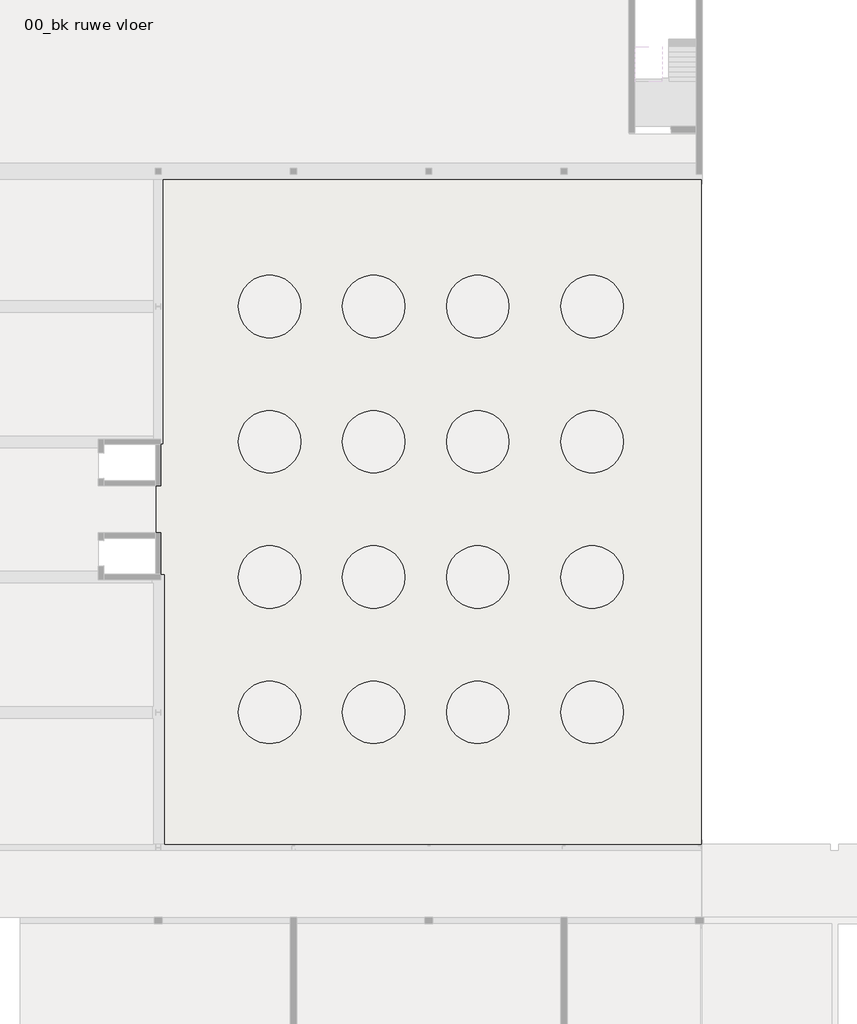
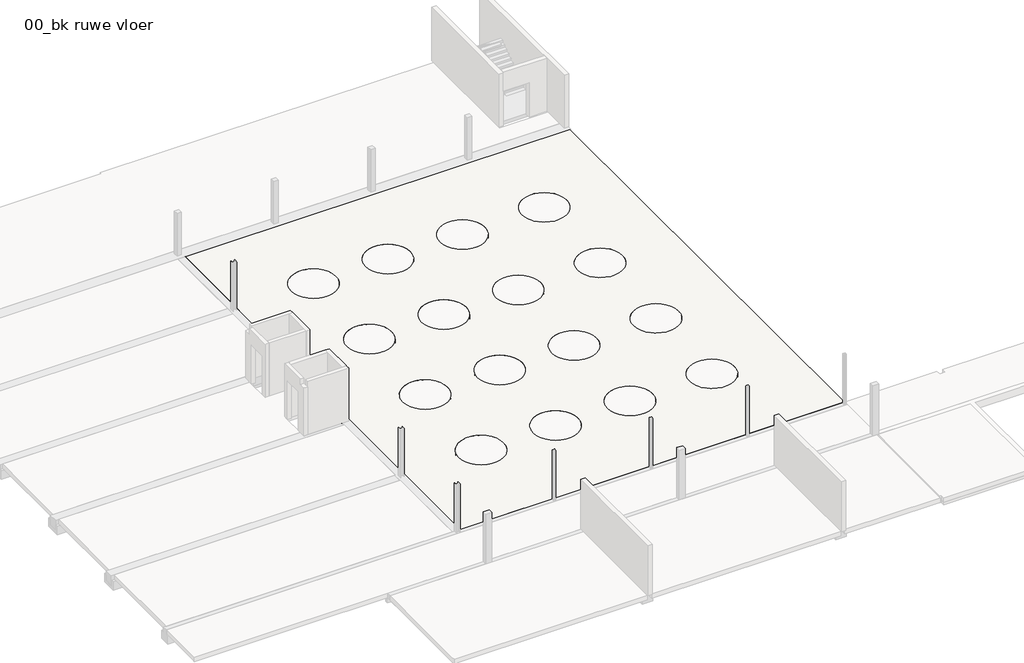
# One storey, part 2 of 6: 2 slabs.
"""IFC4 building model written with IfcOpenShell, lengths in millimetres."""

import ifcopenshell
import ifcopenshell.guid

model = None  # the IFC model being written
_history = None  # IfcOwnerHistory: only IFC2X3 demands one
_inside = {}  # id of a spatial element -> (the spatial element, [elements in it])
_under = {}  # id of a project, library or spatial element -> (it, [spatial elements below it])
_declared = {}  # id of a project -> (the project, [libraries it declares])
_typed = {}  # id of a type object -> (the type object, [elements of that type])
_made_of = {}  # id of a material, layer set ... -> (it, [elements and type objects made of it])


def new_model(schema):
    """Start an empty IFC model of exactly this schema.

    Asked for "IFC4X3", IfcOpenShell would pick the latest addendum, in which some entities
    have other attributes; the version numbers below select the first issue.
    IFC2X3 requires an IfcOwnerHistory on every rooted entity: one is made here for all.
    """
    global model, _history
    if schema == "IFC4X3":
        model = ifcopenshell.file(schema_version=(4, 3, 0, 0))
    else:
        model = ifcopenshell.file(schema=schema)
    _inside.clear()
    _under.clear()
    _declared.clear()
    _typed.clear()
    _made_of.clear()
    _history = None
    if model.schema == "IFC2X3":
        org = make("IfcOrganization", Name="unknown")
        user = make(
            "IfcPersonAndOrganization",
            ThePerson=make("IfcPerson", FamilyName="unknown"),
            TheOrganization=org,
        )
        app = make(
            "IfcApplication",
            ApplicationDeveloper=org,
            Version="unknown",
            ApplicationFullName="unknown",
            ApplicationIdentifier="unknown",
        )
        _history = make(
            "IfcOwnerHistory",
            OwningUser=user,
            OwningApplication=app,
            ChangeAction="ADDED",
            CreationDate=0,
        )
    return model


def make(cls, **values):
    """One entity of the class cls with the attributes given. An attribute that is None is left unset."""
    return model.create_entity(
        cls, **{name: value for name, value in values.items() if value is not None}
    )


def rooted(cls, **values):
    """An entity with a GlobalId (a new one), such as an element, a storey or a relation."""
    return make(cls, GlobalId=ifcopenshell.guid.new(), OwnerHistory=_history, **values)


def si_unit(unit_type, name, prefix=None):
    """IfcSIUnit, for example si_unit("LENGTHUNIT", "METRE", prefix="MILLI")."""
    return make("IfcSIUnit", UnitType=unit_type, Prefix=prefix, Name=name)


def assignment(units):
    """IfcUnitAssignment: the units of a project."""
    return None if units is None else make("IfcUnitAssignment", Units=units)


def point(xyz):
    """IfcCartesianPoint."""
    return None if xyz is None else make("IfcCartesianPoint", Coordinates=xyz)


def direction(xyz):
    """IfcDirection."""
    return None if xyz is None else make("IfcDirection", DirectionRatios=xyz)


def frame(location, z_axis=None, x_axis=None):
    """IfcAxis2Placement3D, a coordinate frame: its origin and axes. An axis left out is left unset."""
    return make(
        "IfcAxis2Placement3D",
        Location=point(location),
        Axis=direction(z_axis),
        RefDirection=direction(x_axis),
    )


def frame_2d(location, x_axis=None):
    """IfcAxis2Placement2D, a coordinate frame in the plane: its origin and x axis."""
    return make(
        "IfcAxis2Placement2D", Location=point(location), RefDirection=direction(x_axis)
    )


def origin():
    """The frame at (0, 0, 0) with its axes left unset."""
    return frame((0.0, 0.0, 0.0))


def place(relative_to, where):
    """IfcLocalPlacement: puts the frame where relative to a parent placement (None: the world)."""
    return make(
        "IfcLocalPlacement", PlacementRelTo=relative_to, RelativePlacement=where
    )


def context(
    kind, dimensions, precision=None, world=None, true_north=None, identifier=None
):
    """IfcGeometricRepresentationContext, for example the 3D "Model" context."""
    return make(
        "IfcGeometricRepresentationContext",
        ContextIdentifier=identifier,
        ContextType=kind,
        CoordinateSpaceDimension=dimensions,
        Precision=precision,
        WorldCoordinateSystem=world,
        TrueNorth=true_north,
    )


def project(units=None, contexts=None):
    """IfcProject with its units and contexts."""
    return rooted(
        "IfcProject",
        Name="project",
        RepresentationContexts=contexts,
        UnitsInContext=assignment(units),
    )


def spatial(cls, under=None, at=None, **own):
    """A site, building, storey or space (cls), placed at a placement, below another one or the project."""
    s = rooted(cls, ObjectPlacement=at, **own)
    if under is not None:
        _under.setdefault(under.id(), (under, []))[1].append(s)
    return s


def polyline(points):
    """IfcPolyline through the points."""
    return make("IfcPolyline", Points=[point(p) for p in points])


def circle_curve(where, radius):
    """IfcCircle in the frame where."""
    return make("IfcCircle", Position=where, Radius=radius)


def trimmed(basis, trim1, trim2, sense, master):
    """IfcTrimmedCurve: the piece of a basis curve between two trims."""
    return make(
        "IfcTrimmedCurve",
        BasisCurve=basis,
        Trim1=trim1,
        Trim2=trim2,
        SenseAgreement=sense,
        MasterRepresentation=master,
    )


def segment(curve, same_sense, transition):
    """IfcCompositeCurveSegment."""
    return make(
        "IfcCompositeCurveSegment",
        Transition=transition,
        SameSense=same_sense,
        ParentCurve=curve,
    )


def composite_curve(segments, self_intersect=None):
    """IfcCompositeCurve: segments joined end to end."""
    return make("IfcCompositeCurve", Segments=segments, SelfIntersect=self_intersect)


def outline(outer, holes=None, kind="AREA"):
    """IfcArbitraryClosedProfileDef: a profile drawn as a closed curve; with holes, ...WithVoids."""
    if holes is None:
        return make("IfcArbitraryClosedProfileDef", ProfileType=kind, OuterCurve=outer)
    return make(
        "IfcArbitraryProfileDefWithVoids",
        ProfileType=kind,
        OuterCurve=outer,
        InnerCurves=holes,
    )


def extrude(swept, where, along, depth):
    """IfcExtrudedAreaSolid: the profile swept, set in the frame where, extruded along a direction by depth."""
    return make(
        "IfcExtrudedAreaSolid",
        SweptArea=swept,
        Position=where,
        ExtrudedDirection=direction(along),
        Depth=depth,
    )


def shape(context_of_items, identifier, shape_type, items):
    """IfcShapeRepresentation: the items that make up one representation, for example the "Body"."""
    return make(
        "IfcShapeRepresentation",
        ContextOfItems=context_of_items,
        RepresentationIdentifier=identifier,
        RepresentationType=shape_type,
        Items=items,
    )


def made_of(thing, what):
    """Note that an element or type object is made of a material, layer set ...; save() writes the relation."""
    if what is not None:
        _made_of.setdefault(what.id(), (what, []))[1].append(thing)
    return thing


def element(
    cls,
    number,
    at=None,
    inside=None,
    cuts=None,
    type_object=None,
    material=None,
    context=None,
    identifier="Body",
    shape_type=None,
    held_by="IfcProductDefinitionShape",
    body=None,
    shapes=None,
    **own,
):
    """One element of the class cls, such as IfcWall. Its Tag is "e" and its number.

    at: its placement. inside: the storey or other place that contains it. cuts: it is an
    opening in that element (IfcRelVoidsElement). A single representation is given by context,
    identifier, shape_type and body (its items); several are given by shapes. held_by: the class
    of the entity that holds the representations. save() writes the other relations.
    """
    e = rooted(cls, Tag="e%d" % number, ObjectPlacement=at, **own)
    if body is not None:
        shapes = [shape(context, identifier, shape_type, body)]
    if shapes is not None:
        e.Representation = make(held_by, Representations=shapes)
    if inside is not None:
        _inside.setdefault(inside.id(), (inside, []))[1].append(e)
    if cuts is not None:
        rooted(
            "IfcRelVoidsElement", RelatingBuildingElement=cuts, RelatedOpeningElement=e
        )
    if type_object is not None:
        _typed.setdefault(type_object.id(), (type_object, []))[1].append(e)
    return made_of(e, material)


def aggregate(whole, parts):
    """IfcRelAggregates: a whole, such as a stair, and the parts it consists of."""
    return rooted("IfcRelAggregates", RelatingObject=whole, RelatedObjects=parts)


def save(model, path):
    """Write the relations noted so far, then the file.

    IfcRelAggregates (storeys below a building ...), IfcRelContainedInSpatialStructure (elements
    in a storey), IfcRelDefinesByType, IfcRelAssociatesMaterial and IfcRelDeclares: one each for
    every whole, place, type object, material and project.
    """
    for whole, parts in _under.values():
        aggregate(whole, parts)
    for where, things in _inside.values():
        rooted(
            "IfcRelContainedInSpatialStructure",
            RelatedElements=things,
            RelatingStructure=where,
        )
    for kind, things in _typed.values():
        rooted("IfcRelDefinesByType", RelatedObjects=things, RelatingType=kind)
    for what, things in _made_of.values():
        rooted("IfcRelAssociatesMaterial", RelatedObjects=things, RelatingMaterial=what)
    for by, libraries in _declared.values():
        rooted("IfcRelDeclares", RelatingContext=by, RelatedDefinitions=libraries)
    model.write(path)


def plane_surface(at):
    """IfcPlane: the flat surface through the origin of the frame at, square to its z axis."""
    return make("IfcPlane", Position=at)


def revolved_surface(curve, axis_point, axis_direction):
    """IfcSurfaceOfRevolution: the curve turned about the line through axis_point along axis_direction."""
    return make(
        "IfcSurfaceOfRevolution",
        SweptCurve=make("IfcArbitraryOpenProfileDef", ProfileType="CURVE", Curve=curve),
        AxisPosition=make("IfcAxis1Placement", Location=point(axis_point), Axis=direction(axis_direction)),
    )


def advanced_brep(points, edges, surfaces, faces):
    """IfcAdvancedBrep: a solid bounded by faces that lie on surfaces and meet in shared edges.

    An edge is (start, end): straight between two places in points (the first is 0);
    or (start, end, curve); or (start, end, curve, False) where it runs against its curve.
    A face is (place in surfaces, loops), or (place, loops, False) where it looks against
    its surface's normal. A loop lists edges by number (the first is 1), with a minus sign
    where the edge is run from its end to its start. The first loop is the outer one.
    """
    corners = [point(p) for p in points]
    vertices = [make("IfcVertexPoint", VertexGeometry=c) for c in corners]
    made = []
    for start, end, *more in edges:
        made.append(
            make(
                "IfcEdgeCurve",
                EdgeStart=vertices[start],
                EdgeEnd=vertices[end],
                EdgeGeometry=more[0] if more else make("IfcPolyline", Points=[corners[start], corners[end]]),
                SameSense=more[1] if len(more) > 1 else True,
            )
        )
    hull = []
    for where, loops, *sense in faces:
        bounds = []
        for j, loop in enumerate(loops):
            ring = [make("IfcOrientedEdge", EdgeElement=made[abs(k) - 1], Orientation=k > 0) for k in loop]
            bounds.append(
                make(
                    "IfcFaceOuterBound" if j == 0 else "IfcFaceBound",
                    Bound=make("IfcEdgeLoop", EdgeList=ring),
                    Orientation=True,
                )
            )
        hull.append(make("IfcAdvancedFace", Bounds=bounds, FaceSurface=surfaces[where], SameSense=sense[0] if sense else True))
    return make("IfcAdvancedBrep", Outer=make("IfcClosedShell", CfsFaces=hull))


model = new_model("IFC4")

# Units and contexts
model_context = context("Model", 3, world=origin())
ifc_project = project(units=[si_unit("LENGTHUNIT", "METRE", prefix="MILLI")], contexts=[model_context])

# Site, building, storey
site = spatial("IfcSite", under=ifc_project)
building = spatial("IfcBuilding", under=site)
storey = spatial("IfcBuildingStorey", under=building, Name="00_bk ruwe vloer", Elevation=-70.0)

# Slabs
placement = place(None, origin())
element("IfcSlab", 1, ObjectType="NLRS_23_FL_breedplaat 320_gen_rsf", at=placement, inside=storey, context=model_context, shape_type="AdvancedBrep", body=[
    advanced_brep(
    [(26250.0, 30375.0, -390.0), (26250.0, 43100.0, -390.0), (52090.0, 43100.0, -390.0), (52090.0, 42900.0, -390.0), (52090.0, 11350.0, -390.0), (52090.0, 11150.0, -390.0), (26300.0, 11150.0, -390.0), (26300.0, 24125.0, -390.0), (25875.0, 24125.0, -390.0), (25875.0, 30375.0, -390.0), (51875.0, 42925.0, -390.0), (26425.0, 42925.0, -390.0), (26425.0, 30365.0, -390.0), (26100.0, 30365.0, -390.0), (26100.0, 28400.0, -390.0), (25885.0, 28400.0, -390.0), (25885.0, 26100.0, -390.0), (26100.0, 26100.0, -390.0), (26100.0, 24135.0, -390.0), (26425.0, 24135.0, -390.0), (26425.0, 11325.0, -390.0), (51875.0, 11325.0, -390.0), (26250.0, 43100.0, -70.0), (26250.0, 30375.0, -70.0), (25875.0, 30375.0, -70.0), (25875.0, 24125.0, -70.0), (26300.0, 24125.0, -70.0), (26300.0, 11150.0, -70.0), (52090.0, 11150.0, -70.0), (52090.0, 43100.0, -70.0), (34850.0, 37000.0, -70.0), (37850.0, 37000.0, -70.0), (45350.0, 37000.0, -70.0), (48350.0, 37000.0, -70.0), (45350.0, 30500.0, -70.0), (48350.0, 30500.0, -70.0), (34850.0, 30500.0, -70.0), (37850.0, 30500.0, -70.0), (34850.0, 24000.0, -70.0), (37850.0, 24000.0, -70.0), (45350.0, 24000.0, -70.0), (48350.0, 24000.0, -70.0), (45350.0, 17500.0, -70.0), (48350.0, 17500.0, -70.0), (34850.0, 17500.0, -70.0), (37850.0, 17500.0, -70.0), (39850.0, 37000.0, -70.0), (42850.0, 37000.0, -70.0), (39850.0, 30500.0, -70.0), (42850.0, 30500.0, -70.0), (39850.0, 24000.0, -70.0), (42850.0, 24000.0, -70.0), (39850.0, 17500.0, -70.0), (42850.0, 17500.0, -70.0), (29850.0, 37000.0, -70.0), (32850.0, 37000.0, -70.0), (29850.0, 30500.0, -70.0), (32850.0, 30500.0, -70.0), (29850.0, 24000.0, -70.0), (32850.0, 24000.0, -70.0), (29850.0, 17500.0, -70.0), (32850.0, 17500.0, -70.0), (34850.0, 37000.0, -330.0), (37850.0, 37000.0, -330.0), (45350.0, 37000.0, -330.0), (48350.0, 37000.0, -330.0), (45350.0, 30500.0, -330.0), (48350.0, 30500.0, -330.0), (34850.0, 30500.0, -330.0), (37850.0, 30500.0, -330.0), (34850.0, 24000.0, -330.0), (37850.0, 24000.0, -330.0), (45350.0, 24000.0, -330.0), (48350.0, 24000.0, -330.0), (45350.0, 17500.0, -330.0), (48350.0, 17500.0, -330.0), (34850.0, 17500.0, -330.0), (37850.0, 17500.0, -330.0), (39850.0, 37000.0, -330.0), (42850.0, 37000.0, -330.0), (39850.0, 30500.0, -330.0), (42850.0, 30500.0, -330.0), (39850.0, 24000.0, -330.0), (42850.0, 24000.0, -330.0), (39850.0, 17500.0, -330.0), (42850.0, 17500.0, -330.0), (29850.0, 37000.0, -330.0), (32850.0, 37000.0, -330.0), (29850.0, 30500.0, -330.0), (32850.0, 30500.0, -330.0), (29850.0, 24000.0, -330.0), (32850.0, 24000.0, -330.0), (29850.0, 17500.0, -330.0), (32850.0, 17500.0, -330.0), (26425.0, 30365.0, -330.0), (26425.0, 42925.0, -330.0), (51875.0, 42925.0, -330.0), (51875.0, 11325.0, -330.0), (26425.0, 11325.0, -330.0), (26425.0, 24135.0, -330.0), (26100.0, 24135.0, -330.0), (26100.0, 26100.0, -330.0), (25885.0, 26100.0, -330.0), (25885.0, 28400.0, -330.0), (26100.0, 28400.0, -330.0), (26100.0, 30365.0, -330.0)],
    [
        (0, 1),
        (1, 2),
        (2, 3),
        (3, 4),
        (4, 5),
        (5, 6),
        (6, 7),
        (7, 8),
        (8, 9),
        (9, 0),
        (10, 11),
        (11, 12),
        (12, 13),
        (13, 14),
        (14, 15),
        (15, 16),
        (16, 17),
        (17, 18),
        (18, 19),
        (19, 20),
        (20, 21),
        (21, 10),
        (22, 23),
        (23, 24),
        (24, 25),
        (25, 26),
        (26, 27),
        (27, 28),
        (28, 29),
        (29, 22),
        (30, 31, circle_curve(frame((36350.0, 37000.0, -70.0), z_axis=(0.0, 0.0, -1.0), x_axis=(1.0, 0.0, 0.0)), 1500.0)),
        (31, 30, circle_curve(frame((36350.0, 37000.0, -70.0), z_axis=(0.0, 0.0, -1.0), x_axis=(1.0, 0.0, 0.0)), 1500.0)),
        (32, 33, circle_curve(frame((46850.0, 37000.0, -70.0), z_axis=(0.0, 0.0, -1.0), x_axis=(1.0, 0.0, 0.0)), 1500.0)),
        (33, 32, circle_curve(frame((46850.0, 37000.0, -70.0), z_axis=(0.0, 0.0, -1.0), x_axis=(1.0, 0.0, 0.0)), 1500.0)),
        (34, 35, circle_curve(frame((46850.0, 30500.0, -70.0), z_axis=(0.0, 0.0, -1.0), x_axis=(1.0, 0.0, 0.0)), 1500.0)),
        (35, 34, circle_curve(frame((46850.0, 30500.0, -70.0), z_axis=(0.0, 0.0, -1.0), x_axis=(1.0, 0.0, 0.0)), 1500.0)),
        (36, 37, circle_curve(frame((36350.0, 30500.0, -70.0), z_axis=(0.0, 0.0, -1.0), x_axis=(1.0, 0.0, 0.0)), 1500.0)),
        (37, 36, circle_curve(frame((36350.0, 30500.0, -70.0), z_axis=(0.0, 0.0, -1.0), x_axis=(1.0, 0.0, 0.0)), 1500.0)),
        (38, 39, circle_curve(frame((36350.0, 24000.0, -70.0), z_axis=(0.0, 0.0, -1.0), x_axis=(1.0, 0.0, 0.0)), 1500.0)),
        (39, 38, circle_curve(frame((36350.0, 24000.0, -70.0), z_axis=(0.0, 0.0, -1.0), x_axis=(1.0, 0.0, 0.0)), 1500.0)),
        (40, 41, circle_curve(frame((46850.0, 24000.0, -70.0), z_axis=(0.0, 0.0, -1.0), x_axis=(1.0, 0.0, 0.0)), 1500.0)),
        (41, 40, circle_curve(frame((46850.0, 24000.0, -70.0), z_axis=(0.0, 0.0, -1.0), x_axis=(1.0, 0.0, 0.0)), 1500.0)),
        (42, 43, circle_curve(frame((46850.0, 17500.0, -70.0), z_axis=(0.0, 0.0, -1.0), x_axis=(1.0, 0.0, 0.0)), 1500.0)),
        (43, 42, circle_curve(frame((46850.0, 17500.0, -70.0), z_axis=(0.0, 0.0, -1.0), x_axis=(1.0, 0.0, 0.0)), 1500.0)),
        (44, 45, circle_curve(frame((36350.0, 17500.0, -70.0), z_axis=(0.0, 0.0, -1.0), x_axis=(1.0, 0.0, 0.0)), 1500.0)),
        (45, 44, circle_curve(frame((36350.0, 17500.0, -70.0), z_axis=(0.0, 0.0, -1.0), x_axis=(1.0, 0.0, 0.0)), 1500.0)),
        (46, 47, circle_curve(frame((41350.0, 37000.0, -70.0), z_axis=(0.0, 0.0, -1.0), x_axis=(1.0, 0.0, 0.0)), 1500.0)),
        (47, 46, circle_curve(frame((41350.0, 37000.0, -70.0), z_axis=(0.0, 0.0, -1.0), x_axis=(1.0, 0.0, 0.0)), 1500.0)),
        (48, 49, circle_curve(frame((41350.0, 30500.0, -70.0), z_axis=(0.0, 0.0, -1.0), x_axis=(1.0, 0.0, 0.0)), 1500.0)),
        (49, 48, circle_curve(frame((41350.0, 30500.0, -70.0), z_axis=(0.0, 0.0, -1.0), x_axis=(1.0, 0.0, 0.0)), 1500.0)),
        (50, 51, circle_curve(frame((41350.0, 24000.0, -70.0), z_axis=(0.0, 0.0, -1.0), x_axis=(1.0, 0.0, 0.0)), 1500.0)),
        (51, 50, circle_curve(frame((41350.0, 24000.0, -70.0), z_axis=(0.0, 0.0, -1.0), x_axis=(1.0, 0.0, 0.0)), 1500.0)),
        (52, 53, circle_curve(frame((41350.0, 17500.0, -70.0), z_axis=(0.0, 0.0, -1.0), x_axis=(1.0, 0.0, 0.0)), 1500.0)),
        (53, 52, circle_curve(frame((41350.0, 17500.0, -70.0), z_axis=(0.0, 0.0, -1.0), x_axis=(1.0, 0.0, 0.0)), 1500.0)),
        (54, 55, circle_curve(frame((31350.0, 37000.0, -70.0), z_axis=(0.0, 0.0, -1.0), x_axis=(1.0, 0.0, 0.0)), 1500.0)),
        (55, 54, circle_curve(frame((31350.0, 37000.0, -70.0), z_axis=(0.0, 0.0, -1.0), x_axis=(1.0, 0.0, 0.0)), 1500.0)),
        (56, 57, circle_curve(frame((31350.0, 30500.0, -70.0), z_axis=(0.0, 0.0, -1.0), x_axis=(1.0, 0.0, 0.0)), 1500.0)),
        (57, 56, circle_curve(frame((31350.0, 30500.0, -70.0), z_axis=(0.0, 0.0, -1.0), x_axis=(1.0, 0.0, 0.0)), 1500.0)),
        (58, 59, circle_curve(frame((31350.0, 24000.0, -70.0), z_axis=(0.0, 0.0, -1.0), x_axis=(1.0, 0.0, 0.0)), 1500.0)),
        (59, 58, circle_curve(frame((31350.0, 24000.0, -70.0), z_axis=(0.0, 0.0, -1.0), x_axis=(1.0, 0.0, 0.0)), 1500.0)),
        (60, 61, circle_curve(frame((31350.0, 17500.0, -70.0), z_axis=(0.0, 0.0, -1.0), x_axis=(1.0, 0.0, 0.0)), 1500.0)),
        (61, 60, circle_curve(frame((31350.0, 17500.0, -70.0), z_axis=(0.0, 0.0, -1.0), x_axis=(1.0, 0.0, 0.0)), 1500.0)),
        (0, 23),
        (22, 1),
        (29, 2),
        (28, 5),
        (27, 6),
        (26, 7),
        (25, 8),
        (24, 9),
        (30, 62),
        (62, 63, circle_curve(frame((36350.0, 37000.0, -330.0), z_axis=(0.0, 0.0, -1.0), x_axis=(1.0, 0.0, 0.0)), 1500.0)),
        (63, 31),
        (63, 62, circle_curve(frame((36350.0, 37000.0, -330.0), z_axis=(0.0, 0.0, -1.0), x_axis=(1.0, 0.0, 0.0)), 1500.0)),
        (32, 64),
        (64, 65, circle_curve(frame((46850.0, 37000.0, -330.0), z_axis=(0.0, 0.0, -1.0), x_axis=(1.0, 0.0, 0.0)), 1500.0)),
        (65, 33),
        (65, 64, circle_curve(frame((46850.0, 37000.0, -330.0), z_axis=(0.0, 0.0, -1.0), x_axis=(1.0, 0.0, 0.0)), 1500.0)),
        (34, 66),
        (66, 67, circle_curve(frame((46850.0, 30500.0, -330.0), z_axis=(0.0, 0.0, -1.0), x_axis=(1.0, 0.0, 0.0)), 1500.0)),
        (67, 35),
        (67, 66, circle_curve(frame((46850.0, 30500.0, -330.0), z_axis=(0.0, 0.0, -1.0), x_axis=(1.0, 0.0, 0.0)), 1500.0)),
        (36, 68),
        (68, 69, circle_curve(frame((36350.0, 30500.0, -330.0), z_axis=(0.0, 0.0, -1.0), x_axis=(1.0, 0.0, 0.0)), 1500.0)),
        (69, 37),
        (69, 68, circle_curve(frame((36350.0, 30500.0, -330.0), z_axis=(0.0, 0.0, -1.0), x_axis=(1.0, 0.0, 0.0)), 1500.0)),
        (38, 70),
        (70, 71, circle_curve(frame((36350.0, 24000.0, -330.0), z_axis=(0.0, 0.0, -1.0), x_axis=(1.0, 0.0, 0.0)), 1500.0)),
        (71, 39),
        (71, 70, circle_curve(frame((36350.0, 24000.0, -330.0), z_axis=(0.0, 0.0, -1.0), x_axis=(1.0, 0.0, 0.0)), 1500.0)),
        (40, 72),
        (72, 73, circle_curve(frame((46850.0, 24000.0, -330.0), z_axis=(0.0, 0.0, -1.0), x_axis=(1.0, 0.0, 0.0)), 1500.0)),
        (73, 41),
        (73, 72, circle_curve(frame((46850.0, 24000.0, -330.0), z_axis=(0.0, 0.0, -1.0), x_axis=(1.0, 0.0, 0.0)), 1500.0)),
        (42, 74),
        (74, 75, circle_curve(frame((46850.0, 17500.0, -330.0), z_axis=(0.0, 0.0, -1.0), x_axis=(1.0, 0.0, 0.0)), 1500.0)),
        (75, 43),
        (75, 74, circle_curve(frame((46850.0, 17500.0, -330.0), z_axis=(0.0, 0.0, -1.0), x_axis=(1.0, 0.0, 0.0)), 1500.0)),
        (44, 76),
        (76, 77, circle_curve(frame((36350.0, 17500.0, -330.0), z_axis=(0.0, 0.0, -1.0), x_axis=(1.0, 0.0, 0.0)), 1500.0)),
        (77, 45),
        (77, 76, circle_curve(frame((36350.0, 17500.0, -330.0), z_axis=(0.0, 0.0, -1.0), x_axis=(1.0, 0.0, 0.0)), 1500.0)),
        (46, 78),
        (78, 79, circle_curve(frame((41350.0, 37000.0, -330.0), z_axis=(0.0, 0.0, -1.0), x_axis=(1.0, 0.0, 0.0)), 1500.0)),
        (79, 47),
        (79, 78, circle_curve(frame((41350.0, 37000.0, -330.0), z_axis=(0.0, 0.0, -1.0), x_axis=(1.0, 0.0, 0.0)), 1500.0)),
        (48, 80),
        (80, 81, circle_curve(frame((41350.0, 30500.0, -330.0), z_axis=(0.0, 0.0, -1.0), x_axis=(1.0, 0.0, 0.0)), 1500.0)),
        (81, 49),
        (81, 80, circle_curve(frame((41350.0, 30500.0, -330.0), z_axis=(0.0, 0.0, -1.0), x_axis=(1.0, 0.0, 0.0)), 1500.0)),
        (50, 82),
        (82, 83, circle_curve(frame((41350.0, 24000.0, -330.0), z_axis=(0.0, 0.0, -1.0), x_axis=(1.0, 0.0, 0.0)), 1500.0)),
        (83, 51),
        (83, 82, circle_curve(frame((41350.0, 24000.0, -330.0), z_axis=(0.0, 0.0, -1.0), x_axis=(1.0, 0.0, 0.0)), 1500.0)),
        (52, 84),
        (84, 85, circle_curve(frame((41350.0, 17500.0, -330.0), z_axis=(0.0, 0.0, -1.0), x_axis=(1.0, 0.0, 0.0)), 1500.0)),
        (85, 53),
        (85, 84, circle_curve(frame((41350.0, 17500.0, -330.0), z_axis=(0.0, 0.0, -1.0), x_axis=(1.0, 0.0, 0.0)), 1500.0)),
        (54, 86),
        (86, 87, circle_curve(frame((31350.0, 37000.0, -330.0), z_axis=(0.0, 0.0, -1.0), x_axis=(1.0, 0.0, 0.0)), 1500.0)),
        (87, 55),
        (87, 86, circle_curve(frame((31350.0, 37000.0, -330.0), z_axis=(0.0, 0.0, -1.0), x_axis=(1.0, 0.0, 0.0)), 1500.0)),
        (56, 88),
        (88, 89, circle_curve(frame((31350.0, 30500.0, -330.0), z_axis=(0.0, 0.0, -1.0), x_axis=(1.0, 0.0, 0.0)), 1500.0)),
        (89, 57),
        (89, 88, circle_curve(frame((31350.0, 30500.0, -330.0), z_axis=(0.0, 0.0, -1.0), x_axis=(1.0, 0.0, 0.0)), 1500.0)),
        (58, 90),
        (90, 91, circle_curve(frame((31350.0, 24000.0, -330.0), z_axis=(0.0, 0.0, -1.0), x_axis=(1.0, 0.0, 0.0)), 1500.0)),
        (91, 59),
        (91, 90, circle_curve(frame((31350.0, 24000.0, -330.0), z_axis=(0.0, 0.0, -1.0), x_axis=(1.0, 0.0, 0.0)), 1500.0)),
        (60, 92),
        (92, 93, circle_curve(frame((31350.0, 17500.0, -330.0), z_axis=(0.0, 0.0, -1.0), x_axis=(1.0, 0.0, 0.0)), 1500.0)),
        (93, 61),
        (93, 92, circle_curve(frame((31350.0, 17500.0, -330.0), z_axis=(0.0, 0.0, -1.0), x_axis=(1.0, 0.0, 0.0)), 1500.0)),
        (94, 95),
        (95, 96),
        (96, 97),
        (97, 98),
        (98, 99),
        (99, 100),
        (100, 101),
        (101, 102),
        (102, 103),
        (103, 104),
        (104, 105),
        (105, 94),
        (95, 11),
        (10, 96),
        (21, 97),
        (20, 98),
        (94, 12),
        (19, 99),
        (18, 100),
        (17, 101),
        (16, 102),
        (15, 103),
        (14, 104),
        (13, 105),
    ],
    [
        plane_surface(frame((26300.0, 24125.0, -390.0), z_axis=(0.0, 0.0, -1.0), x_axis=(0.0, 1.0, 0.0))),
        plane_surface(frame((26300.0, 24125.0, -70.0), z_axis=(0.0, 0.0, 1.0), x_axis=(0.0, -1.0, 0.0))),
        plane_surface(frame((26250.0, 30375.0, -390.0), z_axis=(-1.0, 0.0, 0.0), x_axis=(0.0, 0.0, 1.0))),
        plane_surface(frame((26250.0, 43100.0, -390.0), z_axis=(0.0, 1.0, 0.0), x_axis=(0.0, 0.0, 1.0))),
        plane_surface(frame((52090.0, 43100.0, -390.0), z_axis=(1.0, 0.0, 0.0), x_axis=(0.0, 0.0, 1.0))),
        plane_surface(frame((52090.0, 11150.0, -390.0), z_axis=(0.0, -1.0, 0.0), x_axis=(0.0, 0.0, 1.0))),
        plane_surface(frame((26300.0, 11150.0, -390.0), z_axis=(-1.0, 0.0, 0.0), x_axis=(0.0, 0.0, 1.0))),
        plane_surface(frame((26300.0, 24125.0, -390.0), z_axis=(0.0, -1.0, 0.0), x_axis=(0.0, 0.0, 1.0))),
        plane_surface(frame((25875.0, 24125.0, -390.0), z_axis=(-1.0, 0.0, 0.0), x_axis=(0.0, 0.0, 1.0))),
        plane_surface(frame((25875.0, 30375.0, -390.0), z_axis=(0.0, 1.0, 0.0), x_axis=(0.0, 0.0, 1.0))),
        revolved_surface(polyline([(37850.0, 37000.0, -330.0), (37850.0, 37000.0, -70.0)]), (36350.0, 37000.0, -70.0), (0.0, 0.0, -1.0)),
        revolved_surface(polyline([(48350.0, 37000.0, -330.0), (48350.0, 37000.0, -70.0)]), (46850.0, 37000.0, -70.0), (0.0, 0.0, -1.0)),
        revolved_surface(polyline([(48350.0, 30500.0, -330.0), (48350.0, 30500.0, -70.0)]), (46850.0, 30500.0, -70.0), (0.0, 0.0, -1.0)),
        revolved_surface(polyline([(37850.0, 30500.0, -330.0), (37850.0, 30500.0, -70.0)]), (36350.0, 30500.0, -70.0), (0.0, 0.0, -1.0)),
        revolved_surface(polyline([(37850.0, 24000.0, -330.0), (37850.0, 24000.0, -70.0)]), (36350.0, 24000.0, -70.0), (0.0, 0.0, -1.0)),
        revolved_surface(polyline([(48350.0, 24000.0, -330.0), (48350.0, 24000.0, -70.0)]), (46850.0, 24000.0, -70.0), (0.0, 0.0, -1.0)),
        revolved_surface(polyline([(48350.0, 17500.0, -330.0), (48350.0, 17500.0, -70.0)]), (46850.0, 17500.0, -70.0), (0.0, 0.0, -1.0)),
        revolved_surface(polyline([(37850.0, 17500.0, -330.0), (37850.0, 17500.0, -70.0)]), (36350.0, 17500.0, -70.0), (0.0, 0.0, -1.0)),
        revolved_surface(polyline([(42850.0, 37000.0, -330.0), (42850.0, 37000.0, -70.0)]), (41350.0, 37000.0, -70.0), (0.0, 0.0, -1.0)),
        revolved_surface(polyline([(42850.0, 30500.0, -330.0), (42850.0, 30500.0, -70.0)]), (41350.0, 30500.0, -70.0), (0.0, 0.0, -1.0)),
        revolved_surface(polyline([(42850.0, 24000.0, -330.0), (42850.0, 24000.0, -70.0)]), (41350.0, 24000.0, -70.0), (0.0, 0.0, -1.0)),
        revolved_surface(polyline([(42850.0, 17500.0, -330.0), (42850.0, 17500.0, -70.0)]), (41350.0, 17500.0, -70.0), (0.0, 0.0, -1.0)),
        revolved_surface(polyline([(32850.0, 37000.0, -330.0), (32850.0, 37000.0, -70.0)]), (31350.0, 37000.0, -70.0), (0.0, 0.0, -1.0)),
        revolved_surface(polyline([(32850.0, 30500.0, -330.0), (32850.0, 30500.0, -70.0)]), (31350.0, 30500.0, -70.0), (0.0, 0.0, -1.0)),
        revolved_surface(polyline([(32850.0, 24000.0, -330.0), (32850.0, 24000.0, -70.0)]), (31350.0, 24000.0, -70.0), (0.0, 0.0, -1.0)),
        revolved_surface(polyline([(32850.0, 17500.0, -330.0), (32850.0, 17500.0, -70.0)]), (31350.0, 17500.0, -70.0), (0.0, 0.0, -1.0)),
        plane_surface(frame((51875.0, 42925.0, -330.0), z_axis=(0.0, 0.0, -1.0), x_axis=(-1.0, 0.0, 0.0))),
        plane_surface(frame((26425.0, 42925.0, -390.0), z_axis=(0.0, -1.0, 0.0), x_axis=(0.0, 0.0, 1.0))),
        plane_surface(frame((51875.0, 42925.0, -390.0), z_axis=(-1.0, 0.0, 0.0), x_axis=(0.0, 0.0, 1.0))),
        plane_surface(frame((51875.0, 11325.0, -390.0), z_axis=(0.0, 1.0, 0.0), x_axis=(0.0, 0.0, 1.0))),
        plane_surface(frame((26425.0, 30365.0, -390.0), z_axis=(1.0, 0.0, 0.0), x_axis=(0.0, 0.0, 1.0))),
        plane_surface(frame((26425.0, 11325.0, -390.0), z_axis=(1.0, 0.0, 0.0), x_axis=(0.0, 0.0, 1.0))),
        plane_surface(frame((26425.0, 24135.0, -390.0), z_axis=(0.0, 1.0, 0.0), x_axis=(0.0, 0.0, 1.0))),
        plane_surface(frame((26100.0, 24135.0, -390.0), z_axis=(1.0, 0.0, 0.0), x_axis=(0.0, 0.0, 1.0))),
        plane_surface(frame((26100.0, 26100.0, -390.0), z_axis=(0.0, 1.0, 0.0), x_axis=(0.0, 0.0, 1.0))),
        plane_surface(frame((25885.0, 26100.0, -390.0), z_axis=(1.0, 0.0, 0.0), x_axis=(0.0, 0.0, 1.0))),
        plane_surface(frame((25885.0, 28400.0, -390.0), z_axis=(0.0, -1.0, 0.0), x_axis=(0.0, 0.0, 1.0))),
        plane_surface(frame((26100.0, 28400.0, -390.0), z_axis=(1.0, 0.0, 0.0), x_axis=(0.0, 0.0, 1.0))),
        plane_surface(frame((26100.0, 30365.0, -390.0), z_axis=(0.0, -1.0, 0.0), x_axis=(0.0, 0.0, 1.0))),
    ],
    [
        (0, [[1, 2, 3, 4, 5, 6, 7, 8, 9, 10], [11, 12, 13, 14, 15, 16, 17, 18, 19, 20, 21, 22]]),
        (1, [[23, 24, 25, 26, 27, 28, 29, 30], [31, 32], [33, 34], [35, 36], [37, 38], [39, 40], [41, 42], [43, 44], [45, 46], [47, 48], [49, 50], [51, 52], [53, 54], [55, 56], [57, 58], [59, 60], [61, 62]]),
        (2, [[-1, 63, -23, 64]]),
        (3, [[-2, -64, -30, 65]]),
        (4, [[-5, -4, -3, -65, -29, 66]]),
        (5, [[-6, -66, -28, 67]]),
        (6, [[-7, -67, -27, 68]]),
        (7, [[-8, -68, -26, 69]]),
        (8, [[-9, -69, -25, 70]]),
        (9, [[-10, -70, -24, -63]]),
        (10, [[-31, 71, 72, 73]]),
        (10, [[-32, -73, 74, -71]]),
        (11, [[-33, 75, 76, 77]]),
        (11, [[-34, -77, 78, -75]]),
        (12, [[-35, 79, 80, 81]]),
        (12, [[-36, -81, 82, -79]]),
        (13, [[-37, 83, 84, 85]]),
        (13, [[-38, -85, 86, -83]]),
        (14, [[-39, 87, 88, 89]]),
        (14, [[-40, -89, 90, -87]]),
        (15, [[-41, 91, 92, 93]]),
        (15, [[-42, -93, 94, -91]]),
        (16, [[-43, 95, 96, 97]]),
        (16, [[-44, -97, 98, -95]]),
        (17, [[-45, 99, 100, 101]]),
        (17, [[-46, -101, 102, -99]]),
        (18, [[-47, 103, 104, 105]]),
        (18, [[-48, -105, 106, -103]]),
        (19, [[-49, 107, 108, 109]]),
        (19, [[-50, -109, 110, -107]]),
        (20, [[-51, 111, 112, 113]]),
        (20, [[-52, -113, 114, -111]]),
        (21, [[-53, 115, 116, 117]]),
        (21, [[-54, -117, 118, -115]]),
        (22, [[-55, 119, 120, 121]]),
        (22, [[-56, -121, 122, -119]]),
        (23, [[-57, 123, 124, 125]]),
        (23, [[-58, -125, 126, -123]]),
        (24, [[-59, 127, 128, 129]]),
        (24, [[-60, -129, 130, -127]]),
        (25, [[-61, 131, 132, 133]]),
        (25, [[-62, -133, 134, -131]]),
        (26, [[135, 136, 137, 138, 139, 140, 141, 142, 143, 144, 145, 146], [-72, -74], [-76, -78], [-80, -82], [-84, -86], [-88, -90], [-92, -94], [-96, -98], [-100, -102], [-104, -106], [-108, -110], [-112, -114], [-116, -118], [-120, -122], [-124, -126], [-128, -130], [-132, -134]]),
        (27, [[-136, 147, -11, 148]]),
        (28, [[-137, -148, -22, 149]]),
        (29, [[-138, -149, -21, 150]]),
        (30, [[-135, 151, -12, -147]]),
        (31, [[-139, -150, -20, 152]]),
        (32, [[-140, -152, -19, 153]]),
        (33, [[-141, -153, -18, 154]]),
        (34, [[-142, -154, -17, 155]]),
        (35, [[-143, -155, -16, 156]]),
        (36, [[-144, -156, -15, 157]]),
        (37, [[-145, -157, -14, 158]]),
        (38, [[-146, -158, -13, -151]]),
    ],
),
])
element("IfcSlab", 2, ObjectType="NLRS_23_FL_breedplaat schil 60_gen_rsf", at=placement, inside=storey, context=model_context, shape_type="SweptSolid", body=[
    extrude(outline(polyline([(26425.0, 42925.0), (51875.0, 42925.0), (51875.0, 11325.0), (26425.0, 11325.0), (26425.0, 24135.0), (26100.0, 24135.0), (26100.0, 26100.0), (25885.0, 26100.0), (25885.0, 28400.0), (26100.0, 28400.0), (26100.0, 30365.0), (26425.0, 30365.0), (26425.0, 42925.0)]), holes=[composite_curve([segment(trimmed(circle_curve(frame_2d((31350.0, 37000.0)), 1475.0), [point((29875.0, 37000.0))], [point((32825.0, 37000.0))], True, "CARTESIAN"), True, "CONTINUOUS"), segment(trimmed(circle_curve(frame_2d((31350.0, 37000.0)), 1475.0), [point((32825.0, 37000.0))], [point((29875.0, 37000.0))], True, "CARTESIAN"), True, "CONTINUOUS")], self_intersect=False), composite_curve([segment(trimmed(circle_curve(frame_2d((36350.0, 37000.0)), 1475.0), [point((34875.0, 37000.0))], [point((37825.0, 37000.0))], True, "CARTESIAN"), True, "CONTINUOUS"), segment(trimmed(circle_curve(frame_2d((36350.0, 37000.0)), 1475.0), [point((37825.0, 37000.0))], [point((34875.0, 37000.0))], True, "CARTESIAN"), True, "CONTINUOUS")], self_intersect=False), composite_curve([segment(trimmed(circle_curve(frame_2d((41350.0, 37000.0)), 1475.0), [point((39875.0, 37000.0))], [point((42825.0, 37000.0))], True, "CARTESIAN"), True, "CONTINUOUS"), segment(trimmed(circle_curve(frame_2d((41350.0, 37000.0)), 1475.0), [point((42825.0, 37000.0))], [point((39875.0, 37000.0))], True, "CARTESIAN"), True, "CONTINUOUS")], self_intersect=False), composite_curve([segment(trimmed(circle_curve(frame_2d((46850.0, 37000.0)), 1475.0), [point((45375.0, 37000.0))], [point((48325.0, 37000.0))], True, "CARTESIAN"), True, "CONTINUOUS"), segment(trimmed(circle_curve(frame_2d((46850.0, 37000.0)), 1475.0), [point((48325.0, 37000.0))], [point((45375.0, 37000.0))], True, "CARTESIAN"), True, "CONTINUOUS")], self_intersect=False), composite_curve([segment(trimmed(circle_curve(frame_2d((31350.0, 30500.0)), 1475.0), [point((29875.0, 30500.0))], [point((32825.0, 30500.0))], True, "CARTESIAN"), True, "CONTINUOUS"), segment(trimmed(circle_curve(frame_2d((31350.0, 30500.0)), 1475.0), [point((32825.0, 30500.0))], [point((29875.0, 30500.0))], True, "CARTESIAN"), True, "CONTINUOUS")], self_intersect=False), composite_curve([segment(trimmed(circle_curve(frame_2d((36350.0, 30500.0)), 1475.0), [point((34875.0, 30500.0))], [point((37825.0, 30500.0))], True, "CARTESIAN"), True, "CONTINUOUS"), segment(trimmed(circle_curve(frame_2d((36350.0, 30500.0)), 1475.0), [point((37825.0, 30500.0))], [point((34875.0, 30500.0))], True, "CARTESIAN"), True, "CONTINUOUS")], self_intersect=False), composite_curve([segment(trimmed(circle_curve(frame_2d((41350.0, 30500.0)), 1475.0), [point((39875.0, 30500.0))], [point((42825.0, 30500.0))], True, "CARTESIAN"), True, "CONTINUOUS"), segment(trimmed(circle_curve(frame_2d((41350.0, 30500.0)), 1475.0), [point((42825.0, 30500.0))], [point((39875.0, 30500.0))], True, "CARTESIAN"), True, "CONTINUOUS")], self_intersect=False), composite_curve([segment(trimmed(circle_curve(frame_2d((46850.0, 30500.0)), 1475.0), [point((45375.0, 30500.0))], [point((48325.0, 30500.0))], True, "CARTESIAN"), True, "CONTINUOUS"), segment(trimmed(circle_curve(frame_2d((46850.0, 30500.0)), 1475.0), [point((48325.0, 30500.0))], [point((45375.0, 30500.0))], True, "CARTESIAN"), True, "CONTINUOUS")], self_intersect=False), composite_curve([segment(trimmed(circle_curve(frame_2d((46850.0, 24000.0)), 1475.0), [point((45375.0, 24000.0))], [point((48325.0, 24000.0))], True, "CARTESIAN"), True, "CONTINUOUS"), segment(trimmed(circle_curve(frame_2d((46850.0, 24000.0)), 1475.0), [point((48325.0, 24000.0))], [point((45375.0, 24000.0))], True, "CARTESIAN"), True, "CONTINUOUS")], self_intersect=False), composite_curve([segment(trimmed(circle_curve(frame_2d((41350.0, 24000.0)), 1475.0), [point((39875.0, 24000.0))], [point((42825.0, 24000.0))], True, "CARTESIAN"), True, "CONTINUOUS"), segment(trimmed(circle_curve(frame_2d((41350.0, 24000.0)), 1475.0), [point((42825.0, 24000.0))], [point((39875.0, 24000.0))], True, "CARTESIAN"), True, "CONTINUOUS")], self_intersect=False), composite_curve([segment(trimmed(circle_curve(frame_2d((36350.0, 24000.0)), 1475.0), [point((34875.0, 24000.0))], [point((37825.0, 24000.0))], True, "CARTESIAN"), True, "CONTINUOUS"), segment(trimmed(circle_curve(frame_2d((36350.0, 24000.0)), 1475.0), [point((37825.0, 24000.0))], [point((34875.0, 24000.0))], True, "CARTESIAN"), True, "CONTINUOUS")], self_intersect=False), composite_curve([segment(trimmed(circle_curve(frame_2d((31350.0, 24000.0)), 1475.0), [point((29875.0, 24000.0))], [point((32825.0, 24000.0))], True, "CARTESIAN"), True, "CONTINUOUS"), segment(trimmed(circle_curve(frame_2d((31350.0, 24000.0)), 1475.0), [point((32825.0, 24000.0))], [point((29875.0, 24000.0))], True, "CARTESIAN"), True, "CONTINUOUS")], self_intersect=False), composite_curve([segment(trimmed(circle_curve(frame_2d((31350.0, 17500.0)), 1475.0), [point((29875.0, 17500.0))], [point((32825.0, 17500.0))], True, "CARTESIAN"), True, "CONTINUOUS"), segment(trimmed(circle_curve(frame_2d((31350.0, 17500.0)), 1475.0), [point((32825.0, 17500.0))], [point((29875.0, 17500.0))], True, "CARTESIAN"), True, "CONTINUOUS")], self_intersect=False), composite_curve([segment(trimmed(circle_curve(frame_2d((36350.0, 17500.0)), 1475.0), [point((34875.0, 17500.0))], [point((37825.0, 17500.0))], True, "CARTESIAN"), True, "CONTINUOUS"), segment(trimmed(circle_curve(frame_2d((36350.0, 17500.0)), 1475.0), [point((37825.0, 17500.0))], [point((34875.0, 17500.0))], True, "CARTESIAN"), True, "CONTINUOUS")], self_intersect=False), composite_curve([segment(trimmed(circle_curve(frame_2d((41350.0, 17500.0)), 1475.0), [point((39875.0, 17500.0))], [point((42825.0, 17500.0))], True, "CARTESIAN"), True, "CONTINUOUS"), segment(trimmed(circle_curve(frame_2d((41350.0, 17500.0)), 1475.0), [point((42825.0, 17500.0))], [point((39875.0, 17500.0))], True, "CARTESIAN"), True, "CONTINUOUS")], self_intersect=False), composite_curve([segment(trimmed(circle_curve(frame_2d((46850.0, 17500.0)), 1475.0), [point((45375.0, 17500.0))], [point((48325.0, 17500.0))], True, "CARTESIAN"), True, "CONTINUOUS"), segment(trimmed(circle_curve(frame_2d((46850.0, 17500.0)), 1475.0), [point((48325.0, 17500.0))], [point((45375.0, 17500.0))], True, "CARTESIAN"), True, "CONTINUOUS")], self_intersect=False)]), frame((0.0, 0.0, -390.0), z_axis=(0.0, 0.0, 1.0), x_axis=(1.0, 0.0, 0.0)), (0.0, 0.0, 1.0), 60.0),
])

save(model, "model.ifc")

# Revit data of these elements
# Type "NLRS_23_FL_breedplaat 320_gen_rsf"
#   Keynote = ""
#   Type IfcGUID = "1Sps1bgmr0zeLndh498PCM"
#   Type Comments = "d=320mm"
#   Description = "breedplaatvloer, vrijdragend"
#   Assembly Code = "23.21"
#   Type Mark = ""
#   IfcExportAs = "IfcSlab"
#   Function = 1
#   Layers, outside or top first: 320 mm "NLRS_f2_beton ihwg_gen_rsf" (function 1)
# Type "NLRS_23_FL_breedplaat schil 60_gen_rsf"
#   Keynote = ""
#   Type IfcGUID = "3PAoVTCyX39AT9TmkNvccm"
#   Type Comments = "d=60mm"
#   Description = "prefab breedplaatvloer, vrijdragend"
#   Assembly Code = "23.21"
#   Type Mark = ""
#   IfcExportAs = "IfcSlab"
#   Function = 0
#   Layers, outside or top first: 60 mm "NLRS_f2_beton prefab_gen_rsf" (function 1)
# Element 1 (IfcSlab, "NLRS_23_FL_breedplaat 320_gen_rsf")
#   IfcGUID = "2fqjgN40rEBBKvfwcj0Bhs"
#   built-in parameter 1001955 = 1.5708 (stored number, unit not read)
#   Height Offset From Level = 0 mm
#   built-in parameter 1001954 = 1
#   IsExternal = yes
#   LoadBearing = yes
#   Phase Created = NLRS_nieuw
#   Materials on its faces: "NLRS_f2_beton ihwg_gen_rsf"
# Element 2 (IfcSlab, "NLRS_23_FL_breedplaat schil 60_gen_rsf")
#   IfcGUID = "2SW0URilXFEBqkCpwNtD7E"
#   Comments = ""
#   built-in parameter 1001955 = 3.14159 (stored number, unit not read)
#   Height Offset From Level = -260 mm
#   built-in parameter 1001954 = 1
#   IsExternal = yes
#   LoadBearing = yes
#   Phase Created = NLRS_nieuw
#   Materials on its faces: "NLRS_f2_beton prefab_gen_rsf"
# Materials
#   "NLRS_f2_beton ihwg_gen_rsf": class "F - Niet gebakken kunststeen", colour RGB 129 133 118, transparency 0, Keynote = "f2", Manufacturer = "Revit Standards Foundation", URL = "www.revitstandards.org", Description = "beton ihwg", Cost = 0
#   "NLRS_f2_beton prefab_gen_rsf": class "F - Niet gebakken kunststeen", colour RGB 129 133 118, transparency 0, Keynote = "f2", Manufacturer = "Revit Standards Foundation", URL = "www.revitstandards.org", Description = "beton prefab", Cost = 0
